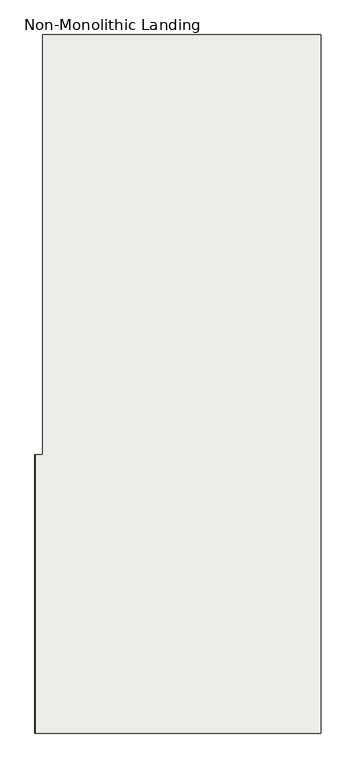
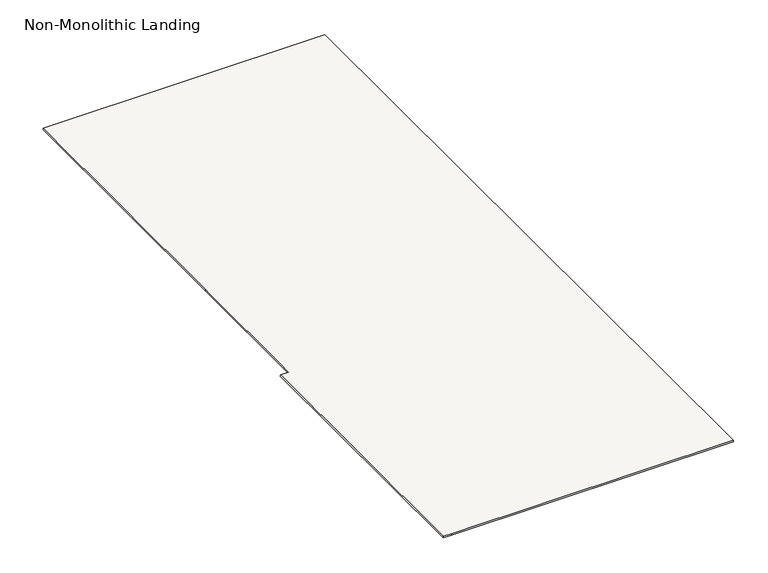
"""IFC4 building model written with IfcOpenShell, lengths in millimetres: slab geometry, Non-Monolithic Landing."""

from ifc_helpers import new_model, si_unit, origin, place, context, project, spatial, faceted_brep, source, transform, mapped, element, save


def non_monolithic_landing_65b4bf74(model_context):
    return source(origin(), model_context, "Body", "Brep", [
        faceted_brep([(-13356.0599092, 11470.4345331, 12058.8235294), (-13356.9099092, 11470.4345331, 12052.8235294), (-13356.9099092, 10370.4345331, 12052.8235294), (-13356.0599092, 10370.4345331, 12058.8235294), (-13325.0, 12030.4345331, 12058.8235294), (-13325.0, 11470.4345331, 12058.8235294), (-13325.0, 10370.4345331, 12058.8235294), (-12225.0, 10370.4345331, 12058.8235294), (-12225.0, 13130.4345331, 12058.8235294), (-13325.0, 13130.4345331, 12058.8235294), (-13325.0, 11470.4345331, 12052.8235294), (-13325.0, 12030.4345331, 12052.8235294), (-13324.15, 12030.4345331, 12052.8235294), (-13324.15, 13130.4345331, 12052.8235294), (-12225.0, 13130.4345331, 12052.8235294), (-12225.0, 10370.4345331, 12052.8235294), (-13325.0, 10370.4345331, 12052.8235294)], [[[0, 1, 2, 3]], [[4, 5, 0, 3, 6, 7, 8, 9]], [[10, 11, 12, 13, 14, 15, 16, 2, 1]], [[5, 4, 11, 10]], [[0, 5, 10, 1]], [[6, 3, 2, 16]], [[7, 6, 16, 15]], [[8, 7, 15, 14]], [[9, 8, 14, 13]], [[4, 12, 11]], [[12, 4, 9, 13]]]),
    ])


if __name__ == "__main__":
    model = new_model("IFC4")
    model_context = context("Model", 3, world=origin())
    ifc_project = project(units=[si_unit("LENGTHUNIT", "METRE", prefix="MILLI")], contexts=[model_context])
    site = spatial("IfcSite", under=ifc_project)
    building = spatial("IfcBuilding", under=site)
    placement = place(None, origin())
    non_monolithic_landing_shape = non_monolithic_landing_65b4bf74(model_context)
    element("IfcSlab", 1, ObjectType="Non-Monolithic Landing", at=placement, inside=building, context=model_context, shape_type="MappedRepresentation", body=[
        mapped(non_monolithic_landing_shape, transform((0.0, 0.0, 0.0), x_axis=(1.0, 0.0, 0.0), y_axis=(0.0, 1.0, 0.0), z_axis=(0.0, 0.0, 1.0))),
    ])
    save(model, "model.ifc")

# Revit data of these elements
# Element 1 (IfcSlab, "Non-Monolithic Landing")
#   Materials on its faces: "Steel, Paint Finish, Dark Gray"
# Materials
#   "Steel, Paint Finish, Dark Gray": class "Metal", colour RGB 89 89 89, transparency 0, Description = "Steel, paint finish, dark gray, glossy", Cost = 0
